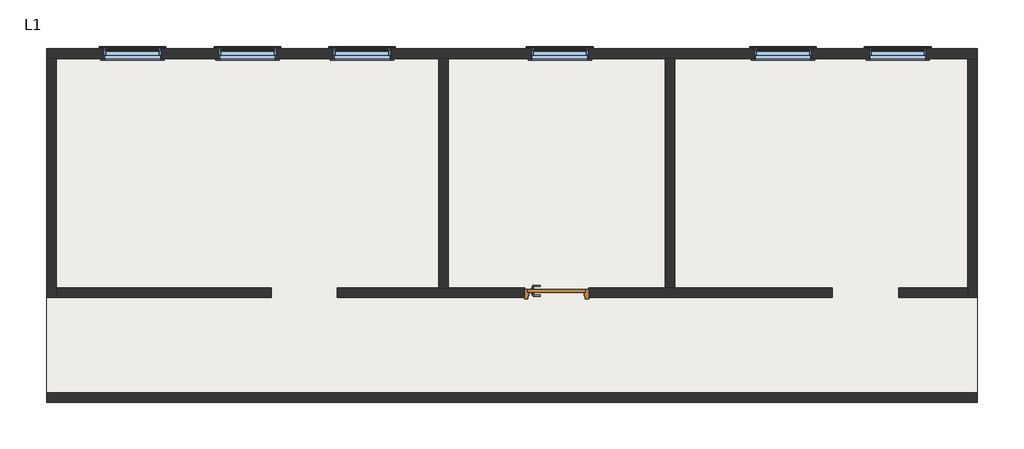
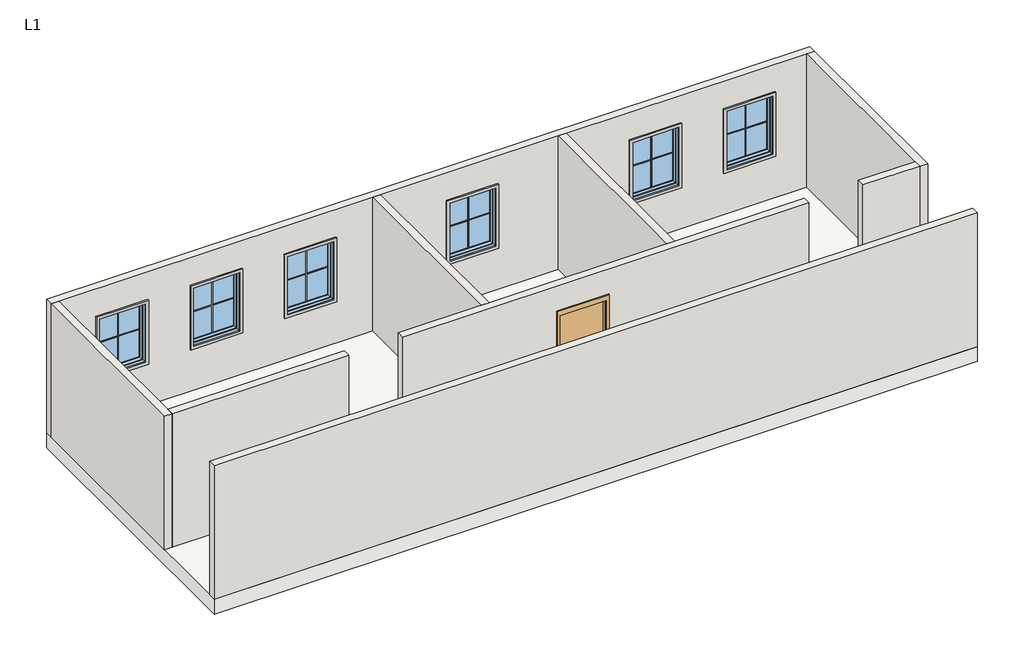
# One storey: 18 proxies, 9 walls, 6 windows, 1 door, 1 slab.
"""IFC4 building model written with IfcOpenShell, lengths in millimetres."""

import ifcopenshell
import ifcopenshell.guid

model = None  # the IFC model being written
_history = None  # IfcOwnerHistory: only IFC2X3 demands one
_inside = {}  # id of a spatial element -> (the spatial element, [elements in it])
_under = {}  # id of a project, library or spatial element -> (it, [spatial elements below it])
_declared = {}  # id of a project -> (the project, [libraries it declares])
_typed = {}  # id of a type object -> (the type object, [elements of that type])
_made_of = {}  # id of a material, layer set ... -> (it, [elements and type objects made of it])


def new_model(schema):
    """Start an empty IFC model of exactly this schema.

    Asked for "IFC4X3", IfcOpenShell would pick the latest addendum, in which some entities
    have other attributes; the version numbers below select the first issue.
    IFC2X3 requires an IfcOwnerHistory on every rooted entity: one is made here for all.
    """
    global model, _history
    if schema == "IFC4X3":
        model = ifcopenshell.file(schema_version=(4, 3, 0, 0))
    else:
        model = ifcopenshell.file(schema=schema)
    _inside.clear()
    _under.clear()
    _declared.clear()
    _typed.clear()
    _made_of.clear()
    _history = None
    if model.schema == "IFC2X3":
        org = make("IfcOrganization", Name="unknown")
        user = make(
            "IfcPersonAndOrganization",
            ThePerson=make("IfcPerson", FamilyName="unknown"),
            TheOrganization=org,
        )
        app = make(
            "IfcApplication",
            ApplicationDeveloper=org,
            Version="unknown",
            ApplicationFullName="unknown",
            ApplicationIdentifier="unknown",
        )
        _history = make(
            "IfcOwnerHistory",
            OwningUser=user,
            OwningApplication=app,
            ChangeAction="ADDED",
            CreationDate=0,
        )
    return model


def make(cls, **values):
    """One entity of the class cls with the attributes given. An attribute that is None is left unset."""
    return model.create_entity(
        cls, **{name: value for name, value in values.items() if value is not None}
    )


def rooted(cls, **values):
    """An entity with a GlobalId (a new one), such as an element, a storey or a relation."""
    return make(cls, GlobalId=ifcopenshell.guid.new(), OwnerHistory=_history, **values)


def si_unit(unit_type, name, prefix=None):
    """IfcSIUnit, for example si_unit("LENGTHUNIT", "METRE", prefix="MILLI")."""
    return make("IfcSIUnit", UnitType=unit_type, Prefix=prefix, Name=name)


def assignment(units):
    """IfcUnitAssignment: the units of a project."""
    return None if units is None else make("IfcUnitAssignment", Units=units)


def point(xyz):
    """IfcCartesianPoint."""
    return None if xyz is None else make("IfcCartesianPoint", Coordinates=xyz)


def direction(xyz):
    """IfcDirection."""
    return None if xyz is None else make("IfcDirection", DirectionRatios=xyz)


def frame(location, z_axis=None, x_axis=None):
    """IfcAxis2Placement3D, a coordinate frame: its origin and axes. An axis left out is left unset."""
    return make(
        "IfcAxis2Placement3D",
        Location=point(location),
        Axis=direction(z_axis),
        RefDirection=direction(x_axis),
    )


def frame_2d(location, x_axis=None):
    """IfcAxis2Placement2D, a coordinate frame in the plane: its origin and x axis."""
    return make(
        "IfcAxis2Placement2D", Location=point(location), RefDirection=direction(x_axis)
    )


def origin():
    """The frame at (0, 0, 0) with its axes left unset."""
    return frame((0.0, 0.0, 0.0))


def origin_with_axes():
    """The frame at (0, 0, 0) with the z axis (0, 0, 1) and the x axis (1, 0, 0) written out."""
    return frame((0.0, 0.0, 0.0), z_axis=(0.0, 0.0, 1.0), x_axis=(1.0, 0.0, 0.0))


def place(relative_to, where):
    """IfcLocalPlacement: puts the frame where relative to a parent placement (None: the world)."""
    return make(
        "IfcLocalPlacement", PlacementRelTo=relative_to, RelativePlacement=where
    )


def context(
    kind, dimensions, precision=None, world=None, true_north=None, identifier=None
):
    """IfcGeometricRepresentationContext, for example the 3D "Model" context."""
    return make(
        "IfcGeometricRepresentationContext",
        ContextIdentifier=identifier,
        ContextType=kind,
        CoordinateSpaceDimension=dimensions,
        Precision=precision,
        WorldCoordinateSystem=world,
        TrueNorth=true_north,
    )


def project(units=None, contexts=None):
    """IfcProject with its units and contexts."""
    return rooted(
        "IfcProject",
        Name="project",
        RepresentationContexts=contexts,
        UnitsInContext=assignment(units),
    )


def spatial(cls, under=None, at=None, **own):
    """A site, building, storey or space (cls), placed at a placement, below another one or the project."""
    s = rooted(cls, ObjectPlacement=at, **own)
    if under is not None:
        _under.setdefault(under.id(), (under, []))[1].append(s)
    return s


def polyline(points):
    """IfcPolyline through the points."""
    return make("IfcPolyline", Points=[point(p) for p in points])


def circle_curve(where, radius):
    """IfcCircle in the frame where."""
    return make("IfcCircle", Position=where, Radius=radius)


def ellipse_curve(where, semi_axis1, semi_axis2):
    """IfcEllipse in the frame where."""
    return make(
        "IfcEllipse", Position=where, SemiAxis1=semi_axis1, SemiAxis2=semi_axis2
    )


def trimmed(basis, trim1, trim2, sense, master):
    """IfcTrimmedCurve: the piece of a basis curve between two trims."""
    return make(
        "IfcTrimmedCurve",
        BasisCurve=basis,
        Trim1=trim1,
        Trim2=trim2,
        SenseAgreement=sense,
        MasterRepresentation=master,
    )


def segment(curve, same_sense, transition):
    """IfcCompositeCurveSegment."""
    return make(
        "IfcCompositeCurveSegment",
        Transition=transition,
        SameSense=same_sense,
        ParentCurve=curve,
    )


def composite_curve(segments, self_intersect=None):
    """IfcCompositeCurve: segments joined end to end."""
    return make("IfcCompositeCurve", Segments=segments, SelfIntersect=self_intersect)


def outline(outer, holes=None, kind="AREA"):
    """IfcArbitraryClosedProfileDef: a profile drawn as a closed curve; with holes, ...WithVoids."""
    if holes is None:
        return make("IfcArbitraryClosedProfileDef", ProfileType=kind, OuterCurve=outer)
    return make(
        "IfcArbitraryProfileDefWithVoids",
        ProfileType=kind,
        OuterCurve=outer,
        InnerCurves=holes,
    )


def extrude(swept, where, along, depth):
    """IfcExtrudedAreaSolid: the profile swept, set in the frame where, extruded along a direction by depth."""
    return make(
        "IfcExtrudedAreaSolid",
        SweptArea=swept,
        Position=where,
        ExtrudedDirection=direction(along),
        Depth=depth,
    )


def faces_of(points, faces, orient=None, outer=None):
    """IfcFace entities. A face is a list of loops; a loop is a list of indices into points, from 0.

    orient and outer hold one flag for each loop. By default every Orientation is true, the
    first loop of a face is its IfcFaceOuterBound and the others are IfcFaceBound.
    """
    made = []
    for i, loops in enumerate(faces):
        bounds = []
        for j, loop in enumerate(loops):
            is_outer = j == 0 if outer is None else outer[i][j]
            bounds.append(
                make(
                    "IfcFaceOuterBound" if is_outer else "IfcFaceBound",
                    Bound=make("IfcPolyLoop", Polygon=[points[k] for k in loop]),
                    Orientation=True if orient is None else orient[i][j],
                )
            )
        made.append(make("IfcFace", Bounds=bounds))
    return made


def faceted_brep(points, faces, orient=None, outer=None, voids=None):
    """IfcFacetedBrep: a solid bounded by flat faces; with voids (closed shells), ...WithVoids."""
    shared = [point(p) for p in points]
    hull = make("IfcClosedShell", CfsFaces=faces_of(shared, faces, orient, outer))
    if voids is None:
        return make("IfcFacetedBrep", Outer=hull)
    return make(
        "IfcFacetedBrepWithVoids",
        Outer=hull,
        Voids=[
            make(cls, CfsFaces=faces_of(shared, fs, o, b)) for cls, fs, o, b in voids
        ],
    )


def shape(context_of_items, identifier, shape_type, items):
    """IfcShapeRepresentation: the items that make up one representation, for example the "Body"."""
    return make(
        "IfcShapeRepresentation",
        ContextOfItems=context_of_items,
        RepresentationIdentifier=identifier,
        RepresentationType=shape_type,
        Items=items,
    )


def source(mapping_origin, context_of_items, identifier, shape_type, items):
    """IfcRepresentationMap: a shape defined once, which mapped items show again and again."""
    return make(
        "IfcRepresentationMap",
        MappingOrigin=mapping_origin,
        MappedRepresentation=shape(context_of_items, identifier, shape_type, items),
    )


def transform(
    local_origin,
    x_axis=None,
    y_axis=None,
    z_axis=None,
    scale=None,
    scale2=None,
    scale3=None,
    uniform=True,
):
    """IfcCartesianTransformationOperator3D, or its non-uniform kind. x_axis, y_axis, z_axis: its Axis1, 2, 3."""
    if uniform:
        return make(
            "IfcCartesianTransformationOperator3D",
            Axis1=direction(x_axis),
            Axis2=direction(y_axis),
            LocalOrigin=point(local_origin),
            Scale=scale,
            Axis3=direction(z_axis),
        )
    return make(
        "IfcCartesianTransformationOperator3DnonUniform",
        Axis1=direction(x_axis),
        Axis2=direction(y_axis),
        LocalOrigin=point(local_origin),
        Scale=scale,
        Axis3=direction(z_axis),
        Scale2=scale2,
        Scale3=scale3,
    )


def mapped(mapping_source, mapping_target):
    """IfcMappedItem: shows the shape of a source again, moved by a transform."""
    return make(
        "IfcMappedItem", MappingSource=mapping_source, MappingTarget=mapping_target
    )


def made_of(thing, what):
    """Note that an element or type object is made of a material, layer set ...; save() writes the relation."""
    if what is not None:
        _made_of.setdefault(what.id(), (what, []))[1].append(thing)
    return thing


def element(
    cls,
    number,
    at=None,
    inside=None,
    cuts=None,
    type_object=None,
    material=None,
    context=None,
    identifier="Body",
    shape_type=None,
    held_by="IfcProductDefinitionShape",
    body=None,
    shapes=None,
    **own,
):
    """One element of the class cls, such as IfcWall. Its Tag is "e" and its number.

    at: its placement. inside: the storey or other place that contains it. cuts: it is an
    opening in that element (IfcRelVoidsElement). A single representation is given by context,
    identifier, shape_type and body (its items); several are given by shapes. held_by: the class
    of the entity that holds the representations. save() writes the other relations.
    """
    e = rooted(cls, Tag="e%d" % number, ObjectPlacement=at, **own)
    if body is not None:
        shapes = [shape(context, identifier, shape_type, body)]
    if shapes is not None:
        e.Representation = make(held_by, Representations=shapes)
    if inside is not None:
        _inside.setdefault(inside.id(), (inside, []))[1].append(e)
    if cuts is not None:
        rooted(
            "IfcRelVoidsElement", RelatingBuildingElement=cuts, RelatedOpeningElement=e
        )
    if type_object is not None:
        _typed.setdefault(type_object.id(), (type_object, []))[1].append(e)
    return made_of(e, material)


def aggregate(whole, parts):
    """IfcRelAggregates: a whole, such as a stair, and the parts it consists of."""
    return rooted("IfcRelAggregates", RelatingObject=whole, RelatedObjects=parts)


def save(model, path):
    """Write the relations noted so far, then the file.

    IfcRelAggregates (storeys below a building ...), IfcRelContainedInSpatialStructure (elements
    in a storey), IfcRelDefinesByType, IfcRelAssociatesMaterial and IfcRelDeclares: one each for
    every whole, place, type object, material and project.
    """
    for whole, parts in _under.values():
        aggregate(whole, parts)
    for where, things in _inside.values():
        rooted(
            "IfcRelContainedInSpatialStructure",
            RelatedElements=things,
            RelatingStructure=where,
        )
    for kind, things in _typed.values():
        rooted("IfcRelDefinesByType", RelatedObjects=things, RelatingType=kind)
    for what, things in _made_of.values():
        rooted("IfcRelAssociatesMaterial", RelatedObjects=things, RelatingMaterial=what)
    for by, libraries in _declared.values():
        rooted("IfcRelDeclares", RelatingContext=by, RelatedDefinitions=libraries)
    model.write(path)


def plane_surface(at):
    """IfcPlane: the flat surface through the origin of the frame at, square to its z axis."""
    return make("IfcPlane", Position=at)


def cylinder_surface(at, radius):
    """IfcCylindricalSurface: all points at the distance radius from the z axis of the frame at."""
    return make("IfcCylindricalSurface", Position=at, Radius=radius)


def revolved_surface(curve, axis_point, axis_direction):
    """IfcSurfaceOfRevolution: the curve turned about the line through axis_point along axis_direction."""
    return make(
        "IfcSurfaceOfRevolution",
        SweptCurve=make("IfcArbitraryOpenProfileDef", ProfileType="CURVE", Curve=curve),
        AxisPosition=make("IfcAxis1Placement", Location=point(axis_point), Axis=direction(axis_direction)),
    )


def advanced_brep(points, edges, surfaces, faces):
    """IfcAdvancedBrep: a solid bounded by faces that lie on surfaces and meet in shared edges.

    An edge is (start, end): straight between two places in points (the first is 0);
    or (start, end, curve); or (start, end, curve, False) where it runs against its curve.
    A face is (place in surfaces, loops), or (place, loops, False) where it looks against
    its surface's normal. A loop lists edges by number (the first is 1), with a minus sign
    where the edge is run from its end to its start. The first loop is the outer one.
    """
    corners = [point(p) for p in points]
    vertices = [make("IfcVertexPoint", VertexGeometry=c) for c in corners]
    made = []
    for start, end, *more in edges:
        made.append(
            make(
                "IfcEdgeCurve",
                EdgeStart=vertices[start],
                EdgeEnd=vertices[end],
                EdgeGeometry=more[0] if more else make("IfcPolyline", Points=[corners[start], corners[end]]),
                SameSense=more[1] if len(more) > 1 else True,
            )
        )
    hull = []
    for where, loops, *sense in faces:
        bounds = []
        for j, loop in enumerate(loops):
            ring = [make("IfcOrientedEdge", EdgeElement=made[abs(k) - 1], Orientation=k > 0) for k in loop]
            bounds.append(
                make(
                    "IfcFaceOuterBound" if j == 0 else "IfcFaceBound",
                    Bound=make("IfcEdgeLoop", EdgeList=ring),
                    Orientation=True,
                )
            )
        hull.append(make("IfcAdvancedFace", Bounds=bounds, FaceSurface=surfaces[where], SameSense=sense[0] if sense else True))
    return make("IfcAdvancedBrep", Outer=make("IfcClosedShell", CfsFaces=hull))


def m_muntin_pattern_2x2_m_muntin_pattern_2x2_ad852c99(model_context):
    return source(origin(), model_context, "Body", "SweptSolid", [
        extrude(outline(polyline([(568.25, -6.35), (568.25, -411.9), (555.55, -411.9), (555.55, -6.35), (0.0, -6.35), (0.0, 6.35), (555.55, 6.35), (555.55, 411.9), (568.25, 411.9), (568.25, 6.35), (1123.8, 6.35), (1123.8, -6.35), (568.25, -6.35)])), frame((0.0, -22.225, 0.0), z_axis=(0.0, 1.0, 0.0), x_axis=(0.0, 0.0, 1.0)), (0.0, 0.0, 1.0), 12.7),
        extrude(outline(polyline([(568.25, -6.35), (568.25, -411.9), (555.55, -411.9), (555.55, -6.35), (0.0, -6.35), (0.0, 6.35), (555.55, 6.35), (555.55, 411.9), (568.25, 411.9), (568.25, 6.35), (1123.8, 6.35), (1123.8, -6.35), (568.25, -6.35)])), frame((0.0, 9.525, 0.0), z_axis=(0.0, 1.0, 0.0), x_axis=(0.0, 0.0, 1.0)), (0.0, 0.0, 1.0), 12.7),
    ])


def m_trim_window_exterior_flat_with_sill_71544b40(model_context):
    return source(origin(), model_context, "Body", "SweptSolid", [
        extrude(outline(polyline([(510.0, -1220.4323709), (510.0, -1280.4323709), (-510.0, -1280.4323709), (-510.0, -1220.4323709), (510.0, -1220.4323709)])), origin_with_axes(), (0.0, 0.0, 1.0), 19.05),
        extrude(outline(polyline([(-1230.0, 38.1), (-1202.4580645, 38.1), (-1200.0, 19.05), (-1200.0, 0.0), (-1220.4323709, 0.0), (-1220.4323709, 19.05), (-1230.0, 19.05), (-1230.0, 38.1)])), frame((-522.7, 0.0, 0.0), z_axis=(1.0, 0.0, 0.0), x_axis=(0.0, 1.0, 0.0)), (0.0, 0.0, 1.0), 1045.4),
        extrude(outline(polyline([(-510.0, 60.0), (510.0, 60.0), (510.0, -1200.0), (450.0, -1200.0), (450.0, 0.0), (-450.0, 0.0), (-450.0, -1200.0), (-510.0, -1200.0), (-510.0, 60.0)])), origin_with_axes(), (0.0, 0.0, 1.0), 19.05),
    ])


def m_trim_window_interior_flat_picture_frame_24fe8ef8(model_context):
    return source(origin(), model_context, "Body", "SweptSolid", [
        extrude(outline(polyline([(497.3, 47.3), (497.3, -1247.3), (-497.3, -1247.3), (-497.3, 47.3), (497.3, 47.3)]), holes=[polyline([(437.3, -12.7), (-437.3, -12.7), (-437.3, -1187.3), (437.3, -1187.3), (437.3, -12.7)])]), origin_with_axes(), (0.0, 0.0, 1.0), 30.0),
    ])


def m_door_passage_single_flush_900_x_2100mm_f70d95c9(model_context):
    return source(origin(), model_context, "Body", "SolidModel", [
        advanced_brep(
        [(-384.990625, 3.35, 1000.0), (-364.990625, 3.35, 1000.0), (-364.990625, -26.65, 1000.0), (-384.990625, -26.65, 1000.0), (-359.990625, -31.65, 1000.0), (-359.990625, -51.65, 1000.0), (-254.990625, -51.65, 1000.0), (-254.990625, -31.65, 1000.0)],
        [
            (0, 1, circle_curve(frame((-374.990625, 3.35, 1000.0), z_axis=(0.0, 1.0, 0.0), x_axis=(1.0, 0.0, 0.0)), 10.0)),
            (1, 0, circle_curve(frame((-374.990625, 3.35, 1000.0), z_axis=(0.0, 1.0, 0.0), x_axis=(1.0, 0.0, 0.0)), 10.0)),
            (1, 2),
            (2, 3, circle_curve(frame((-374.990625, -26.65, 1000.0), z_axis=(0.0, 1.0, 0.0), x_axis=(1.0, 0.0, 0.0)), 10.0)),
            (3, 0),
            (3, 2, circle_curve(frame((-374.990625, -26.65, 1000.0), z_axis=(0.0, 1.0, 0.0), x_axis=(1.0, 0.0, 0.0)), 10.0)),
            (4, 5, circle_curve(frame((-359.990625, -41.65, 1000.0), z_axis=(-1.0, 0.0, 0.0), x_axis=(0.0, 1.0, 0.0)), 10.0)),
            (5, 3, circle_curve(frame((-359.990625, -26.65, 1000.0), z_axis=(0.0, 0.0, -1.0), x_axis=(-1.0, 0.0, 0.0)), 25.0)),
            (2, 4, circle_curve(frame((-359.990625, -26.65, 1000.0), z_axis=(0.0, 0.0, 1.0), x_axis=(-1.0, 0.0, 0.0)), 5.0)),
            (5, 4, circle_curve(frame((-359.990625, -41.65, 1000.0), z_axis=(-1.0, 0.0, 0.0), x_axis=(0.0, 1.0, 0.0)), 10.0)),
            (6, 7, circle_curve(frame((-254.990625, -41.65, 1000.0), z_axis=(1.0, 0.0, 0.0), x_axis=(0.0, 1.0, 0.0)), 10.0)),
            (7, 6, circle_curve(frame((-254.990625, -41.65, 1000.0), z_axis=(1.0, 0.0, 0.0), x_axis=(0.0, 1.0, 0.0)), 10.0)),
            (4, 7),
            (6, 5),
        ],
        [
            plane_surface(frame((-374.990625, 3.35, 1000.0), z_axis=(0.0, 1.0, 0.0), x_axis=(0.0, 0.0, 1.0))),
            cylinder_surface(frame((-374.990625, 3.35, 1000.0), z_axis=(0.0, 1.0, 0.0), x_axis=(1.0, 0.0, 0.0)), 10.0),
            revolved_surface(trimmed(ellipse_curve(frame((-374.990625, -26.65, 1000.0), z_axis=(0.0, -1.0, 0.0), x_axis=(1.0, 0.0, 0.0)), 10.0, 10.0), [point((-384.990625, -26.65, 1000.0))], [point((-364.990625, -26.65, 1000.0))], True, "CARTESIAN"), (-359.990625, -26.65, 1000.0), (0.0, 0.0, -1.0)),
            revolved_surface(trimmed(ellipse_curve(frame((-374.990625, -26.65, 1000.0), z_axis=(0.0, -1.0, 0.0), x_axis=(1.0, 0.0, 0.0)), 10.0, 10.0), [point((-364.990625, -26.65, 1000.0))], [point((-384.990625, -26.65, 1000.0))], True, "CARTESIAN"), (-359.990625, -26.65, 1000.0), (0.0, 0.0, -1.0)),
            plane_surface(frame((-254.990625, -41.65, 1000.0), z_axis=(1.0, 0.0, 0.0), x_axis=(0.0, 0.0, 1.0))),
            cylinder_surface(frame((-359.990625, -41.65, 1000.0), z_axis=(-1.0, 0.0, 0.0), x_axis=(0.0, 1.0, 0.0)), 10.0),
        ],
        [
            (0, [[1, 2]]),
            (1, [[3, 4, 5, -2]]),
            (1, [[-5, 6, -3, -1]]),
            (2, [[7, 8, -4, 9]]),
            (3, [[10, -9, -6, -8]]),
            (4, [[11, 12]]),
            (5, [[13, -11, 14, -7]]),
            (5, [[-14, -12, -13, -10]]),
        ],
    ),
        extrude(outline(composite_curve([segment(trimmed(circle_curve(frame_2d((1000.0, -377.490625)), 30.0), [point((1000.0, -407.490625))], [point((1000.0, -347.490625))], False, "CARTESIAN"), True, "CONTINUOUS"), segment(trimmed(circle_curve(frame_2d((1000.0, -377.490625)), 30.0), [point((1000.0, -347.490625))], [point((1000.0, -407.490625))], False, "CARTESIAN"), True, "CONTINUOUS")], self_intersect=False)), frame((0.0, 3.35, 0.0), z_axis=(0.0, 1.0, 0.0), x_axis=(0.0, 0.0, 1.0)), (0.0, 0.0, 1.0), 8.0),
        advanced_brep(
        [(-384.990625, 64.35, 1000.0), (-364.990625, 64.35, 1000.0), (-384.990625, 94.35, 1000.0), (-364.990625, 94.35, 1000.0), (-359.990625, 99.35, 1000.0), (-359.990625, 119.35, 1000.0), (-254.990625, 119.35, 1000.0), (-254.990625, 99.35, 1000.0)],
        [
            (0, 1, circle_curve(frame((-374.990625, 64.35, 1000.0), z_axis=(0.0, -1.0, 0.0), x_axis=(1.0, 0.0, 0.0)), 10.0)),
            (1, 0, circle_curve(frame((-374.990625, 64.35, 1000.0), z_axis=(0.0, -1.0, 0.0), x_axis=(1.0, 0.0, 0.0)), 10.0)),
            (0, 2),
            (2, 3, circle_curve(frame((-374.990625, 94.35, 1000.0), z_axis=(0.0, -1.0, 0.0), x_axis=(1.0, 0.0, 0.0)), 10.0)),
            (3, 1),
            (3, 2, circle_curve(frame((-374.990625, 94.35, 1000.0), z_axis=(0.0, -1.0, 0.0), x_axis=(1.0, 0.0, 0.0)), 10.0)),
            (4, 3, circle_curve(frame((-359.990625, 94.35, 1000.0), z_axis=(0.0, 0.0, 1.0), x_axis=(-1.0, 0.0, 0.0)), 5.0)),
            (2, 5, circle_curve(frame((-359.990625, 94.35, 1000.0), z_axis=(0.0, 0.0, -1.0), x_axis=(-1.0, 0.0, 0.0)), 25.0)),
            (5, 4, circle_curve(frame((-359.990625, 109.35, 1000.0), z_axis=(-1.0, 0.0, 0.0), x_axis=(0.0, -1.0, 0.0)), 10.0)),
            (4, 5, circle_curve(frame((-359.990625, 109.35, 1000.0), z_axis=(-1.0, 0.0, 0.0), x_axis=(0.0, -1.0, 0.0)), 10.0)),
            (6, 7, circle_curve(frame((-254.990625, 109.35, 1000.0), z_axis=(1.0, 0.0, 0.0), x_axis=(0.0, -1.0, 0.0)), 10.0)),
            (7, 6, circle_curve(frame((-254.990625, 109.35, 1000.0), z_axis=(1.0, 0.0, 0.0), x_axis=(0.0, -1.0, 0.0)), 10.0)),
            (5, 6),
            (7, 4),
        ],
        [
            plane_surface(frame((-374.990625, 64.35, 1000.0), z_axis=(0.0, -1.0, 0.0), x_axis=(0.0, 0.0, 1.0))),
            cylinder_surface(frame((-374.990625, 64.35, 1000.0), z_axis=(0.0, -1.0, 0.0), x_axis=(1.0, 0.0, 0.0)), 10.0),
            revolved_surface(trimmed(ellipse_curve(frame((-374.990625, 94.35, 1000.0), z_axis=(0.0, -1.0, 0.0), x_axis=(1.0, 0.0, 0.0)), 10.0, 10.0), [point((-384.990625, 94.35, 1000.0))], [point((-364.990625, 94.35, 1000.0))], True, "CARTESIAN"), (-359.990625, 94.35, 1000.0), (0.0, 0.0, -1.0)),
            revolved_surface(trimmed(ellipse_curve(frame((-374.990625, 94.35, 1000.0), z_axis=(0.0, -1.0, 0.0), x_axis=(1.0, 0.0, 0.0)), 10.0, 10.0), [point((-364.990625, 94.35, 1000.0))], [point((-384.990625, 94.35, 1000.0))], True, "CARTESIAN"), (-359.990625, 94.35, 1000.0), (0.0, 0.0, -1.0)),
            plane_surface(frame((-254.990625, 109.35, 1000.0), z_axis=(1.0, 0.0, 0.0), x_axis=(0.0, 0.0, 1.0))),
            cylinder_surface(frame((-359.990625, 109.35, 1000.0), z_axis=(-1.0, 0.0, 0.0), x_axis=(0.0, -1.0, 0.0)), 10.0),
        ],
        [
            (0, [[1, 2]]),
            (1, [[-1, 3, 4, 5]]),
            (1, [[-2, -5, 6, -3]]),
            (2, [[7, -4, 8, 9]]),
            (3, [[-8, -6, -7, 10]]),
            (4, [[11, 12]]),
            (5, [[-9, 13, -12, 14]]),
            (5, [[-10, -14, -11, -13]]),
        ],
    ),
        extrude(outline(composite_curve([segment(trimmed(circle_curve(frame_2d((1000.0, -377.490625)), 30.0), [point((1000.0, -407.490625))], [point((1000.0, -347.490625))], False, "CARTESIAN"), True, "CONTINUOUS"), segment(trimmed(circle_curve(frame_2d((1000.0, -377.490625)), 30.0), [point((1000.0, -347.490625))], [point((1000.0, -407.490625))], False, "CARTESIAN"), True, "CONTINUOUS")], self_intersect=False)), frame((0.0, 56.35, 0.0), z_axis=(0.0, 1.0, 0.0), x_axis=(0.0, 0.0, 1.0)), (0.0, 0.0, 1.0), 8.0),
        extrude(outline(polyline([(450.0, 11.35), (-450.0, 11.35), (-450.0, 56.35), (450.0, 56.35), (450.0, 11.35)])), origin_with_axes(), (0.0, 0.0, 1.0), 2100.0),
        faceted_brep([(450.0, 6.5875, 0.0), (450.0, 56.35, 0.0), (500.0, 56.35, 0.0), (500.0, -93.65, 0.0), (450.0, -93.65, 0.0), (450.0, -44.4375, 0.0), (434.125, -44.4375, 0.0), (434.125, 6.5875, 0.0), (450.0, 6.5875, 2100.0), (450.0, 56.35, 2100.0), (-450.0, 56.35, 2100.0), (-450.0, 56.35, 0.0), (-500.0, 56.35, 0.0), (-500.0, 56.35, 2200.0), (500.0, 56.35, 2200.0), (500.0, -93.65, 2200.0), (-500.0, -93.65, 2200.0), (-500.0, -93.65, 0.0), (-450.0, -93.65, 0.0), (-450.0, -93.65, 2100.0), (450.0, -93.65, 2100.0), (450.0, -44.4375, 2100.0), (-450.0, -44.4375, 2100.0), (-450.0, -44.4375, 0.0), (-434.125, -44.4375, 0.0), (-434.125, -44.4375, 2084.125), (434.125, -44.4375, 2084.125), (434.125, 6.5875, 2084.125), (-434.125, 6.5875, 2084.125), (-434.125, 6.5875, 0.0), (-450.0, 6.5875, 0.0), (-450.0, 6.5875, 2100.0)], [[[0, 1, 2, 3, 4, 5, 6, 7]], [[1, 0, 8, 9]], [[2, 1, 9, 10, 11, 12, 13, 14]], [[3, 2, 14, 15]], [[4, 3, 15, 16, 17, 18, 19, 20]], [[5, 4, 20, 21]], [[6, 5, 21, 22, 23, 24, 25, 26]], [[7, 6, 26, 27]], [[0, 7, 27, 28, 29, 30, 31, 8]], [[9, 8, 31, 10]], [[20, 19, 22, 21]], [[26, 25, 28, 27]], [[12, 11, 30, 29, 24, 23, 18, 17]], [[11, 10, 31, 30]], [[13, 12, 17, 16]], [[19, 18, 23, 22]], [[25, 24, 29, 28]], [[15, 14, 13, 16]]]),
    ])


def m_window_fixed_900_x_1200mm_f2c8dc95(model_context):
    return source(origin(), model_context, "Body", "SolidModel", [
        faceted_brep([(450.0, -20.25, 2100.0), (450.0, 94.05, 2100.0), (-450.0, 94.05, 2100.0), (-450.0, -20.25, 2100.0), (-450.0, 94.05, 900.0), (-450.0, -20.25, 900.0), (450.0, 94.05, 900.0), (450.0, -20.25, 900.0), (418.25, -20.25, 2068.25), (418.25, -20.25, 931.75), (-418.25, -20.25, 931.75), (-418.25, -20.25, 2068.25), (-437.3, 94.05, 2087.3), (-437.3, 94.05, 912.7), (437.3, 94.05, 912.7), (437.3, 94.05, 2087.3), (418.25, 43.25, 2068.25), (-418.25, 43.25, 2068.25), (437.3, 43.25, 2087.3), (-437.3, 43.25, 2087.3), (-418.25, 43.25, 931.75), (-437.3, 43.25, 912.7), (418.25, 43.25, 931.75), (437.3, 43.25, 912.7)], [[[0, 1, 2, 3]], [[3, 2, 4, 5]], [[5, 4, 6, 7]], [[3, 5, 7, 0], [8, 9, 10, 11]], [[7, 6, 1, 0]], [[1, 6, 4, 2], [12, 13, 14, 15]], [[16, 8, 11, 17]], [[15, 18, 19, 12]], [[17, 11, 10, 20]], [[12, 19, 21, 13]], [[20, 10, 9, 22]], [[13, 21, 23, 14]], [[22, 9, 8, 16]], [[18, 23, 21, 19], [17, 20, 22, 16]], [[14, 23, 18, 15]]]),
        extrude(outline(polyline([(2100.0, -450.0), (900.0, -450.0), (900.0, 450.0), (2100.0, 450.0), (2100.0, -450.0)]), holes=[polyline([(2087.3, 437.3), (912.7, 437.3), (912.7, -437.3), (2087.3, -437.3), (2087.3, 437.3)])]), frame((0.0, -75.0, 0.0), z_axis=(0.0, 1.0, 0.0), x_axis=(0.0, 0.0, 1.0)), (0.0, 0.0, 1.0), 54.75),
        extrude(outline(polyline([(912.7, 437.3), (2087.3, 437.3), (2087.3, -437.3), (912.7, -437.3), (912.7, 437.3)]), holes=[polyline([(938.1, -411.9), (2061.9, -411.9), (2061.9, 411.9), (938.1, 411.9), (938.1, -411.9)])]), frame((0.0, 43.25, 0.0), z_axis=(0.0, 1.0, 0.0), x_axis=(0.0, 0.0, 1.0)), (0.0, 0.0, 1.0), 44.45),
        extrude(outline(polyline([(411.9, 75.0), (411.9, 68.65), (-411.9, 68.65), (-411.9, 75.0), (411.9, 75.0)])), frame((0.0, 0.0, 938.1), z_axis=(0.0, 0.0, 1.0), x_axis=(1.0, 0.0, 0.0)), (0.0, 0.0, 1.0), 1123.8),
        extrude(outline(polyline([(-411.9, 55.95), (-411.9, 62.3), (411.9, 62.3), (411.9, 55.95), (-411.9, 55.95)])), frame((0.0, 0.0, 938.1), z_axis=(0.0, 0.0, 1.0), x_axis=(1.0, 0.0, 0.0)), (0.0, 0.0, 1.0), 1123.8),
    ])


model = new_model("IFC4")

# Units and contexts
model_context = context("Model", 3, world=origin())
ifc_project = project(units=[si_unit("LENGTHUNIT", "METRE", prefix="MILLI")], contexts=[model_context])

# Site, building, storey
site = spatial("IfcSite", under=ifc_project)
building = spatial("IfcBuilding", under=site)
storey = spatial("IfcBuildingStorey", under=building, Name="L1", Elevation=0.0)

# Proxies
placement = place(None, origin())
m_muntin_pattern_2x2_m_muntin_pattern_2x2_shape = m_muntin_pattern_2x2_m_muntin_pattern_2x2_ad852c99(model_context)
element("IfcBuildingElementProxy", 1, Name="M_Muntin Pattern_2x2 : M_Muntin Pattern_2x2", ObjectType="M_Muntin Pattern_2x2 : M_Muntin Pattern_2x2", at=placement, inside=storey, context=model_context, shape_type="MappedRepresentation", body=[
    mapped(m_muntin_pattern_2x2_m_muntin_pattern_2x2_shape, transform((1675.0, 3815.475, 938.1), x_axis=(-1.0, 0.0, 0.0), y_axis=(0.0, -1.0, 0.0), z_axis=(0.0, 0.0, 1.0))),
])
element("IfcBuildingElementProxy", 2, Name="M_Muntin Pattern_2x2 : M_Muntin Pattern_2x2", ObjectType="M_Muntin Pattern_2x2 : M_Muntin Pattern_2x2", at=placement, inside=storey, context=model_context, shape_type="MappedRepresentation", body=[
    mapped(m_muntin_pattern_2x2_m_muntin_pattern_2x2_shape, transform((-1425.0, 3815.475, 938.1), x_axis=(-1.0, 0.0, 0.0), y_axis=(0.0, -1.0, 0.0), z_axis=(0.0, 0.0, 1.0))),
])
element("IfcBuildingElementProxy", 3, Name="M_Muntin Pattern_2x2 : M_Muntin Pattern_2x2", ObjectType="M_Muntin Pattern_2x2 : M_Muntin Pattern_2x2", at=placement, inside=storey, context=model_context, shape_type="MappedRepresentation", body=[
    mapped(m_muntin_pattern_2x2_m_muntin_pattern_2x2_shape, transform((-3225.0, 3815.475, 938.1), x_axis=(-1.0, 0.0, 0.0), y_axis=(0.0, -1.0, 0.0), z_axis=(0.0, 0.0, 1.0))),
])
element("IfcBuildingElementProxy", 4, Name="M_Muntin Pattern_2x2 : M_Muntin Pattern_2x2", ObjectType="M_Muntin Pattern_2x2 : M_Muntin Pattern_2x2", at=placement, inside=storey, context=model_context, shape_type="MappedRepresentation", body=[
    mapped(m_muntin_pattern_2x2_m_muntin_pattern_2x2_shape, transform((-5025.0, 3815.475, 938.1), x_axis=(-1.0, 0.0, 0.0), y_axis=(0.0, -1.0, 0.0), z_axis=(0.0, 0.0, 1.0))),
])
element("IfcBuildingElementProxy", 5, Name="M_Muntin Pattern_2x2 : M_Muntin Pattern_2x2", ObjectType="M_Muntin Pattern_2x2 : M_Muntin Pattern_2x2", at=placement, inside=storey, context=model_context, shape_type="MappedRepresentation", body=[
    mapped(m_muntin_pattern_2x2_m_muntin_pattern_2x2_shape, transform((5175.0, 3815.475, 938.1), x_axis=(-1.0, 0.0, 0.0), y_axis=(0.0, -1.0, 0.0), z_axis=(0.0, 0.0, 1.0))),
])
element("IfcBuildingElementProxy", 6, Name="M_Muntin Pattern_2x2 : M_Muntin Pattern_2x2", ObjectType="M_Muntin Pattern_2x2 : M_Muntin Pattern_2x2", at=placement, inside=storey, context=model_context, shape_type="MappedRepresentation", body=[
    mapped(m_muntin_pattern_2x2_m_muntin_pattern_2x2_shape, transform((6975.0, 3815.475, 938.1), x_axis=(-1.0, 0.0, 0.0), y_axis=(0.0, -1.0, 0.0), z_axis=(0.0, 0.0, 1.0))),
])
m_trim_window_exterior_flat_with_sill_shape = m_trim_window_exterior_flat_with_sill_71544b40(model_context)
element("IfcBuildingElementProxy", 7, Name="M_Trim-Window-Exterior-Flat : with Sill", ObjectType="M_Trim-Window-Exterior-Flat : with Sill", at=placement, inside=storey, context=model_context, shape_type="MappedRepresentation", body=[
    mapped(m_trim_window_exterior_flat_with_sill_shape, transform((1675.0, 3825.0, 2100.0), x_axis=(-1.0, 0.0, 0.0), y_axis=(0.0, 0.0, 1.0), z_axis=(0.0, 1.0, 0.0))),
])
element("IfcBuildingElementProxy", 8, Name="M_Trim-Window-Exterior-Flat : with Sill", ObjectType="M_Trim-Window-Exterior-Flat : with Sill", at=placement, inside=storey, context=model_context, shape_type="MappedRepresentation", body=[
    mapped(m_trim_window_exterior_flat_with_sill_shape, transform((-1425.0, 3825.0, 2100.0), x_axis=(-1.0, 0.0, 0.0), y_axis=(0.0, 0.0, 1.0), z_axis=(0.0, 1.0, 0.0))),
])
element("IfcBuildingElementProxy", 9, Name="M_Trim-Window-Exterior-Flat : with Sill", ObjectType="M_Trim-Window-Exterior-Flat : with Sill", at=placement, inside=storey, context=model_context, shape_type="MappedRepresentation", body=[
    mapped(m_trim_window_exterior_flat_with_sill_shape, transform((-3225.0, 3825.0, 2100.0), x_axis=(-1.0, 0.0, 0.0), y_axis=(0.0, 0.0, 1.0), z_axis=(0.0, 1.0, 0.0))),
])
element("IfcBuildingElementProxy", 10, Name="M_Trim-Window-Exterior-Flat : with Sill", ObjectType="M_Trim-Window-Exterior-Flat : with Sill", at=placement, inside=storey, context=model_context, shape_type="MappedRepresentation", body=[
    mapped(m_trim_window_exterior_flat_with_sill_shape, transform((-5025.0, 3825.0, 2100.0), x_axis=(-1.0, 0.0, 0.0), y_axis=(0.0, 0.0, 1.0), z_axis=(0.0, 1.0, 0.0))),
])
element("IfcBuildingElementProxy", 11, Name="M_Trim-Window-Exterior-Flat : with Sill", ObjectType="M_Trim-Window-Exterior-Flat : with Sill", at=placement, inside=storey, context=model_context, shape_type="MappedRepresentation", body=[
    mapped(m_trim_window_exterior_flat_with_sill_shape, transform((5175.0, 3825.0, 2100.0), x_axis=(-1.0, 0.0, 0.0), y_axis=(0.0, 0.0, 1.0), z_axis=(0.0, 1.0, 0.0))),
])
element("IfcBuildingElementProxy", 12, Name="M_Trim-Window-Exterior-Flat : with Sill", ObjectType="M_Trim-Window-Exterior-Flat : with Sill", at=placement, inside=storey, context=model_context, shape_type="MappedRepresentation", body=[
    mapped(m_trim_window_exterior_flat_with_sill_shape, transform((6975.0, 3825.0, 2100.0), x_axis=(-1.0, 0.0, 0.0), y_axis=(0.0, 0.0, 1.0), z_axis=(0.0, 1.0, 0.0))),
])
m_trim_window_interior_flat_picture_frame_shape = m_trim_window_interior_flat_picture_frame_24fe8ef8(model_context)
element("IfcBuildingElementProxy", 13, Name="M_Trim-Window-Interior-Flat : Picture Frame", ObjectType="M_Trim-Window-Interior-Flat : Picture Frame", at=placement, inside=storey, context=model_context, shape_type="MappedRepresentation", body=[
    mapped(m_trim_window_interior_flat_picture_frame_shape, transform((1675.0, 3675.0, 2100.0), x_axis=(1.0, 0.0, 0.0), y_axis=(0.0, 0.0, 1.0), z_axis=(0.0, -1.0, 0.0))),
])
element("IfcBuildingElementProxy", 14, Name="M_Trim-Window-Interior-Flat : Picture Frame", ObjectType="M_Trim-Window-Interior-Flat : Picture Frame", at=placement, inside=storey, context=model_context, shape_type="MappedRepresentation", body=[
    mapped(m_trim_window_interior_flat_picture_frame_shape, transform((-1425.0, 3675.0, 2100.0), x_axis=(1.0, 0.0, 0.0), y_axis=(0.0, 0.0, 1.0), z_axis=(0.0, -1.0, 0.0))),
])
element("IfcBuildingElementProxy", 15, Name="M_Trim-Window-Interior-Flat : Picture Frame", ObjectType="M_Trim-Window-Interior-Flat : Picture Frame", at=placement, inside=storey, context=model_context, shape_type="MappedRepresentation", body=[
    mapped(m_trim_window_interior_flat_picture_frame_shape, transform((-3225.0, 3675.0, 2100.0), x_axis=(1.0, 0.0, 0.0), y_axis=(0.0, 0.0, 1.0), z_axis=(0.0, -1.0, 0.0))),
])
element("IfcBuildingElementProxy", 16, Name="M_Trim-Window-Interior-Flat : Picture Frame", ObjectType="M_Trim-Window-Interior-Flat : Picture Frame", at=placement, inside=storey, context=model_context, shape_type="MappedRepresentation", body=[
    mapped(m_trim_window_interior_flat_picture_frame_shape, transform((-5025.0, 3675.0, 2100.0), x_axis=(1.0, 0.0, 0.0), y_axis=(0.0, 0.0, 1.0), z_axis=(0.0, -1.0, 0.0))),
])
element("IfcBuildingElementProxy", 17, Name="M_Trim-Window-Interior-Flat : Picture Frame", ObjectType="M_Trim-Window-Interior-Flat : Picture Frame", at=placement, inside=storey, context=model_context, shape_type="MappedRepresentation", body=[
    mapped(m_trim_window_interior_flat_picture_frame_shape, transform((5175.0, 3675.0, 2100.0), x_axis=(1.0, 0.0, 0.0), y_axis=(0.0, 0.0, 1.0), z_axis=(0.0, -1.0, 0.0))),
])
element("IfcBuildingElementProxy", 18, Name="M_Trim-Window-Interior-Flat : Picture Frame", ObjectType="M_Trim-Window-Interior-Flat : Picture Frame", at=placement, inside=storey, context=model_context, shape_type="MappedRepresentation", body=[
    mapped(m_trim_window_interior_flat_picture_frame_shape, transform((6975.0, 3675.0, 2100.0), x_axis=(1.0, 0.0, 0.0), y_axis=(0.0, 0.0, 1.0), z_axis=(0.0, -1.0, 0.0))),
])

# Door
m_door_passage_single_flush_900_x_2100mm_shape = m_door_passage_single_flush_900_x_2100mm_f70d95c9(model_context)
element("IfcDoor", 19, ObjectType="M_Door-Passage-Single-Flush : 900 x 2100mm", at=placement, inside=storey, context=model_context, shape_type="MappedRepresentation", body=[
    mapped(m_door_passage_single_flush_900_x_2100mm_shape, transform((1625.0, -6.35, 0.0), x_axis=(1.0, 0.0, 0.0), y_axis=(0.0, 1.0, 0.0), z_axis=(0.0, 0.0, 1.0))),
])

# Slab
element("IfcSlab", 20, ObjectType="Generic 300mm", at=placement, inside=storey, context=model_context, shape_type="SweptSolid", body=[
    extrude(outline(polyline([(8225.0, 3825.0), (8225.0, -1725.0), (-6375.0, -1725.0), (-6375.0, 3825.0), (8225.0, 3825.0)])), frame((0.0, 0.0, -300.0), z_axis=(0.0, 0.0, 1.0), x_axis=(1.0, 0.0, 0.0)), (0.0, 0.0, 1.0), 300.0),
])

# Walls
element("IfcWall", 21, ObjectType="Generic - 150mm", at=placement, inside=storey, context=model_context, shape_type="SweptSolid", body=[
    extrude(outline(polyline([(-75.0, 3675.0), (-75.0, 75.0), (-225.0, 75.0), (-225.0, 3675.0), (-75.0, 3675.0)])), origin_with_axes(), (0.0, 0.0, 1.0), 2700.0),
])
element("IfcWall", 22, ObjectType="Generic - 150mm", at=placement, inside=storey, context=model_context, shape_type="Brep", body=[
    faceted_brep([(-6375.0, 3675.0, 0.0), (-6225.0, 3675.0, 0.0), (-225.0, 3675.0, 0.0), (-75.0, 3675.0, 0.0), (3325.0, 3675.0, 0.0), (3475.0, 3675.0, 0.0), (8075.0, 3675.0, 0.0), (8225.0, 3675.0, 0.0), (8225.0, 3675.0, 2700.0), (8075.0, 3675.0, 2700.0), (3475.0, 3675.0, 2700.0), (3325.0, 3675.0, 2700.0), (-75.0, 3675.0, 2700.0), (-225.0, 3675.0, 2700.0), (-6225.0, 3675.0, 2700.0), (-6375.0, 3675.0, 2700.0), (2125.0, 3675.0, 2100.0), (2125.0, 3675.0, 900.0), (1225.0, 3675.0, 900.0), (1225.0, 3675.0, 2100.0), (-975.0, 3675.0, 2100.0), (-975.0, 3675.0, 900.0), (-1875.0, 3675.0, 900.0), (-1875.0, 3675.0, 2100.0), (-2775.0, 3675.0, 2100.0), (-2775.0, 3675.0, 900.0), (-3675.0, 3675.0, 900.0), (-3675.0, 3675.0, 2100.0), (-4575.0, 3675.0, 2100.0), (-4575.0, 3675.0, 900.0), (-5475.0, 3675.0, 900.0), (-5475.0, 3675.0, 2100.0), (5625.0, 3675.0, 2100.0), (5625.0, 3675.0, 900.0), (4725.0, 3675.0, 900.0), (4725.0, 3675.0, 2100.0), (7425.0, 3675.0, 2100.0), (7425.0, 3675.0, 900.0), (6525.0, 3675.0, 900.0), (6525.0, 3675.0, 2100.0), (-6375.0, 3825.0, 0.0), (-6375.0, 3825.0, 2700.0), (8225.0, 3825.0, 2700.0), (8225.0, 3825.0, 0.0), (2125.0, 3825.0, 2100.0), (1225.0, 3825.0, 2100.0), (1225.0, 3825.0, 900.0), (2125.0, 3825.0, 900.0), (-975.0, 3825.0, 2100.0), (-1875.0, 3825.0, 2100.0), (-1875.0, 3825.0, 900.0), (-975.0, 3825.0, 900.0), (-2775.0, 3825.0, 2100.0), (-3675.0, 3825.0, 2100.0), (-3675.0, 3825.0, 900.0), (-2775.0, 3825.0, 900.0), (-4575.0, 3825.0, 2100.0), (-5475.0, 3825.0, 2100.0), (-5475.0, 3825.0, 900.0), (-4575.0, 3825.0, 900.0), (5625.0, 3825.0, 2100.0), (4725.0, 3825.0, 2100.0), (4725.0, 3825.0, 900.0), (5625.0, 3825.0, 900.0), (7425.0, 3825.0, 2100.0), (6525.0, 3825.0, 2100.0), (6525.0, 3825.0, 900.0), (7425.0, 3825.0, 900.0)], [[[0, 1, 2, 3, 4, 5, 6, 7, 8, 9, 10, 11, 12, 13, 14, 15], [16, 17, 18, 19], [20, 21, 22, 23], [24, 25, 26, 27], [28, 29, 30, 31], [32, 33, 34, 35], [36, 37, 38, 39]], [[40, 41, 42, 43], [44, 45, 46, 47], [48, 49, 50, 51], [52, 53, 54, 55], [56, 57, 58, 59], [60, 61, 62, 63], [64, 65, 66, 67]], [[7, 6, 5, 4, 3, 2, 1, 0, 40, 43]], [[15, 14, 13, 12, 11, 10, 9, 8, 42, 41]], [[0, 15, 41, 40]], [[8, 7, 43, 42]], [[17, 16, 44, 47]], [[18, 17, 47, 46]], [[19, 18, 46, 45]], [[16, 19, 45, 44]], [[21, 20, 48, 51]], [[22, 21, 51, 50]], [[23, 22, 50, 49]], [[20, 23, 49, 48]], [[25, 24, 52, 55]], [[26, 25, 55, 54]], [[27, 26, 54, 53]], [[24, 27, 53, 52]], [[29, 28, 56, 59]], [[30, 29, 59, 58]], [[31, 30, 58, 57]], [[28, 31, 57, 56]], [[33, 32, 60, 63]], [[34, 33, 63, 62]], [[35, 34, 62, 61]], [[32, 35, 61, 60]], [[37, 36, 64, 67]], [[38, 37, 67, 66]], [[39, 38, 66, 65]], [[36, 39, 65, 64]]]),
])
element("IfcWall", 23, ObjectType="Generic - 150mm", at=placement, inside=storey, context=model_context, shape_type="SweptSolid", body=[
    extrude(outline(polyline([(3325.0, 75.0), (3325.0, 3675.0), (3475.0, 3675.0), (3475.0, 75.0), (3325.0, 75.0)])), origin_with_axes(), (0.0, 0.0, 1.0), 2700.0),
])
element("IfcWall", 24, ObjectType="Generic - 150mm", at=placement, inside=storey, context=model_context, shape_type="SweptSolid", body=[
    extrude(outline(polyline([(6987.5, 75.0), (8075.0, 75.0), (8075.0, -75.0), (6987.5, -75.0), (6987.5, 75.0)])), origin_with_axes(), (0.0, 0.0, 1.0), 2700.0),
])
element("IfcWall", 25, ObjectType="Generic - 150mm", at=placement, inside=storey, context=model_context, shape_type="Brep", body=[
    faceted_brep([(-6375.0, 3675.0, 0.0), (-6375.0, -75.0, 0.0), (-6375.0, -75.0, 2700.0), (-6375.0, 3675.0, 2700.0), (-6225.0, 3675.0, 0.0), (-6225.0, 3675.0, 2700.0), (-6225.0, 75.0, 2700.0), (-6225.0, -75.0, 2700.0), (-6225.0, -75.0, 0.0), (-6225.0, 75.0, 0.0)], [[[0, 1, 2, 3]], [[4, 5, 6, 7, 8, 9]], [[1, 0, 4, 9, 8]], [[3, 2, 7, 6, 5]], [[0, 3, 5, 4]], [[2, 1, 8, 7]]]),
])
element("IfcWall", 26, ObjectType="Generic - 150mm", at=placement, inside=storey, context=model_context, shape_type="Brep", body=[
    faceted_brep([(8075.0, 3675.0, 0.0), (8075.0, 75.0, 0.0), (8075.0, -75.0, 0.0), (8075.0, -75.0, 2700.0), (8075.0, 75.0, 2700.0), (8075.0, 3675.0, 2700.0), (8225.0, 3675.0, 0.0), (8225.0, 3675.0, 2700.0), (8225.0, -75.0, 2700.0), (8225.0, -75.0, 0.0)], [[[0, 1, 2, 3, 4, 5]], [[6, 7, 8, 9]], [[2, 1, 0, 6, 9]], [[5, 4, 3, 8, 7]], [[0, 5, 7, 6]], [[3, 2, 9, 8]]]),
])
element("IfcWall", 27, ObjectType="Generic - 150mm", at=placement, inside=storey, context=model_context, shape_type="SweptSolid", body=[
    extrude(outline(polyline([(-6375.0, -1575.0), (8225.0, -1575.0), (8225.0, -1725.0), (-6375.0, -1725.0), (-6375.0, -1575.0)])), origin_with_axes(), (0.0, 0.0, 1.0), 2700.0),
])
element("IfcWall", 28, ObjectType="Generic - 150mm", at=placement, inside=storey, context=model_context, shape_type="SweptSolid", body=[
    extrude(outline(polyline([(-6225.0, 75.0), (-2850.0, 75.0), (-2850.0, -75.0), (-6225.0, -75.0), (-6225.0, 75.0)])), origin_with_axes(), (0.0, 0.0, 1.0), 2700.0),
])
element("IfcWall", 29, ObjectType="Generic - 150mm", at=placement, inside=storey, context=model_context, shape_type="Brep", body=[
    faceted_brep([(-1812.5, 75.0, 0.0), (-1812.5, 75.0, 2700.0), (-225.0, 75.0, 2700.0), (-75.0, 75.0, 2700.0), (3325.0, 75.0, 2700.0), (3475.0, 75.0, 2700.0), (5950.0, 75.0, 2700.0), (5950.0, 75.0, 0.0), (3475.0, 75.0, 0.0), (3325.0, 75.0, 0.0), (2125.0, 75.0, 0.0), (2125.0, 75.0, 2200.0), (1125.0, 75.0, 2200.0), (1125.0, 75.0, 0.0), (-75.0, 75.0, 0.0), (-225.0, 75.0, 0.0), (-1812.5, -75.0, 2700.0), (-1812.5, -75.0, 0.0), (1125.0, -75.0, 0.0), (1125.0, -75.0, 2200.0), (2125.0, -75.0, 2200.0), (2125.0, -75.0, 0.0), (5950.0, -75.0, 0.0), (5950.0, -75.0, 2700.0)], [[[0, 1, 2, 3, 4, 5, 6, 7, 8, 9, 10, 11, 12, 13, 14, 15]], [[16, 17, 18, 19, 20, 21, 22, 23]], [[17, 0, 15, 14, 13, 18]], [[7, 22, 21, 10, 9, 8]], [[1, 0, 17, 16]], [[6, 5, 4, 3, 2, 1, 16, 23]], [[7, 6, 23, 22]], [[20, 11, 10, 21]], [[11, 20, 19, 12]], [[12, 19, 18, 13]]]),
])

# Windows
m_window_fixed_900_x_1200mm_shape = m_window_fixed_900_x_1200mm_f2c8dc95(model_context)
element("IfcWindow", 30, ObjectType="M_Window-Fixed : 900 x 1200mm", at=placement, inside=storey, context=model_context, shape_type="MappedRepresentation", body=[
    mapped(m_window_fixed_900_x_1200mm_shape, transform((1675.0, 3750.0, 0.0), x_axis=(1.0, 0.0, 0.0), y_axis=(0.0, 1.0, 0.0), z_axis=(0.0, 0.0, 1.0))),
])
element("IfcWindow", 31, ObjectType="M_Window-Fixed : 900 x 1200mm", at=placement, inside=storey, context=model_context, shape_type="MappedRepresentation", body=[
    mapped(m_window_fixed_900_x_1200mm_shape, transform((-1425.0, 3750.0, 0.0), x_axis=(1.0, 0.0, 0.0), y_axis=(0.0, 1.0, 0.0), z_axis=(0.0, 0.0, 1.0))),
])
element("IfcWindow", 32, ObjectType="M_Window-Fixed : 900 x 1200mm", at=placement, inside=storey, context=model_context, shape_type="MappedRepresentation", body=[
    mapped(m_window_fixed_900_x_1200mm_shape, transform((-3225.0, 3750.0, 0.0), x_axis=(1.0, 0.0, 0.0), y_axis=(0.0, 1.0, 0.0), z_axis=(0.0, 0.0, 1.0))),
])
element("IfcWindow", 33, ObjectType="M_Window-Fixed : 900 x 1200mm", at=placement, inside=storey, context=model_context, shape_type="MappedRepresentation", body=[
    mapped(m_window_fixed_900_x_1200mm_shape, transform((-5025.0, 3750.0, 0.0), x_axis=(1.0, 0.0, 0.0), y_axis=(0.0, 1.0, 0.0), z_axis=(0.0, 0.0, 1.0))),
])
element("IfcWindow", 34, ObjectType="M_Window-Fixed : 900 x 1200mm", at=placement, inside=storey, context=model_context, shape_type="MappedRepresentation", body=[
    mapped(m_window_fixed_900_x_1200mm_shape, transform((5175.0, 3750.0, 0.0), x_axis=(1.0, 0.0, 0.0), y_axis=(0.0, 1.0, 0.0), z_axis=(0.0, 0.0, 1.0))),
])
element("IfcWindow", 35, ObjectType="M_Window-Fixed : 900 x 1200mm", at=placement, inside=storey, context=model_context, shape_type="MappedRepresentation", body=[
    mapped(m_window_fixed_900_x_1200mm_shape, transform((6975.0, 3750.0, 0.0), x_axis=(1.0, 0.0, 0.0), y_axis=(0.0, 1.0, 0.0), z_axis=(0.0, 0.0, 1.0))),
])

save(model, "model.ifc")

# Revit data of these elements
# Project information
#   Organization Name = "Organization Name"
#   Organization Description = "Organization Description"
#   Building Name = "Building Name"
#   Project Issue Date = "Issue Date"
#   Project Status = "Project Status"
#   Client Name = "Client Name"
#   Project Address = "Enter address here\nAddress Line 2"
#   Project Name = "Project Name"
#   Project Number = "Project Number"
# Type "M_Muntin Pattern_2x2 : M_Muntin Pattern_2x2"
#   Width [instance default] = 1200 mm
#   Thickness = 12.7 mm
#   Height [instance default] = 1200 mm
#   Distance = 19.05 mm
#   Interior Material [instance default] = none
#   Exterior Material [instance default] = none
#   Default Elevation = 0
# Type "M_Trim-Window-Exterior-Flat : with Sill"
#   Trim Width = 60 mm
#   Trim Thickness_Picture Frame = 30 mm
#   Trim Thickness_with Sill = 19.05 mm
#   Sill Thickness = 30 mm
#   Opening Width [instance default] = 600 mm
#   Opening Height [instance default] = 900 mm
#   Default Elevation = 1200 mm
#   Sill = yes
#   Picture Frame = no
#   Trim Material [instance default] = none
# Type "M_Trim-Window-Interior-Flat : Picture Frame"
#   Trim Thickness_Picture Frame = 30 mm
#   Trim Width = 60 mm
#   Trim Thickness_with Sill = 20 mm
#   Sill Thickness = 30 mm
#   Opening Width [instance default] = 600 mm
#   Opening Height [instance default] = 900 mm
#   Default Elevation = 1200 mm
#   Sill = no
#   Picture Frame = yes
#   Trim Material [instance default] = none
# Type "M_Door-Passage-Single-Flush : 900 x 2100mm"
#   Type Mark = "38"
#   Analytic Construction = "Wooden"
#   Thickness = 45 mm
#   Thermal Resistance (R) = 0.455703 (m²·K)/W
#   Swing Angle [instance default] = 90.00°
#   Strike Height = 1000 mm
#   Rough Width [instance default] = 1000 mm
#   Rough Height [instance default] = 2200 mm
#   MF Opening Height [instance default] = 100 mm
#   MF Opening Width [instance default] = 100 mm
#   Inset Calculate [instance default] = 105 mm
#   Masonry Inset [instance default] = 25 mm
#   Height = 2100 mm
#   Width = 900 mm
#   Heat Transfer Coefficient (U) = 2.19465 W/(m²·K)
#   Masonry Frame Depth = 150 mm
#   Masonry Frame [instance default] = yes
#   Function = 1
#   Dry Wall Frame [instance default] = no
#   Panel Material = Wood - Birch
#   Frame Material = Metal - Paint Finish - Grey
#   Door Handle Material = Aluminum
#   Visual Light Transmittance = 0
#   Solar Heat Gain Coefficient = 0
#   Wall Closure = (empty or 0)
# Type "Generic 300mm"
#   Description = "Generic Floor (Material By Category), 300mm thick"
#   Function = 0
#   Layers, outside or top first: 300 mm no material (function 1)
# Type "Generic - 150mm"
#   Description = "Generic Wall (Material By Category), 150mm thick"
#   Type Mark = "G04"
#   Layers, outside or top first: 150 mm no material (function 1)
# Type "M_Window-Fixed : 900 x 1200mm"
#   Type Mark = "36"
#   Fire Rating = "0.5h"
#   Analytic Construction = "Double glazing - domestic"
#   Window Inset [instance default] = 0 mm
#   Wall Thickness [instance default] = 150 mm
#   Visual Light Transmittance = 0.81
#   Thermal Resistance (R) = 0.319569 (m²·K)/W
#   Solar Heat Gain Coefficient = 0.76
#   Rough Width = 915 mm
#   Rough Height = 1215 mm
#   Interior Wall Closure [instance default] = 54.75 mm
#   Height = 1200 mm
#   Heat Transfer Coefficient (U) = 3.12929 W/(m²·K)
#   Frame Extension [instance default] = 6.35 mm
#   Exterior Wall Closure [instance default] = 31.75 mm
#   Extension Jamb [instance default] = 54.75 mm
#   Default Sill Height = 900 mm
#   Width = 900 mm
#   Muntin Visibility = yes
#   Interior Trim Visibility [instance default] = yes
#   Exterior Trim Visibility [instance default] = yes
#   Extension Jamb Visibility [instance default] = yes
#   Muntin Pattern = M_Muntin Pattern_2x2 : M_Muntin Pattern_2x2
#   Interior Trim Material = Wood - Stained
#   Interior Trim = M_Trim-Window-Interior-Flat : Picture Frame
#   Interior Frame Material = Wood - Stained
#   Glass Panel Material = Glass
#   Exterior Trim Material = Clad - White
#   Exterior Trim = M_Trim-Window-Exterior-Flat : with Sill
#   Exterior Frame Material = Clad - White
#   Wall Closure = (empty or 0)
# Elements 1, 2, 3, 4, 5, 6 (IfcBuildingElementProxy, "M_Muntin Pattern_2x2 : M_Muntin Pattern_2x2")
#   Width = 823.8 mm
#   Height = 1123.8 mm
#   Interior Material = Wood - Stained
#   Exterior Material = Clad - White
#   Phase Created = New Construction
#   Materials on its faces: "Clad - White", "Wood - Stained"
# Elements 7, 8, 9, 10, 11, 12 (IfcBuildingElementProxy, "M_Trim-Window-Exterior-Flat : with Sill")
#   Opening Width = 900 mm
#   Opening Height = 1200 mm
#   Trim Material = Clad - White
#   Phase Created = New Construction
#   Materials on its faces: "Clad - White"
# Elements 13, 14, 15, 16, 17, 18 (IfcBuildingElementProxy, "M_Trim-Window-Interior-Flat : Picture Frame")
#   Opening Width = 900 mm
#   Opening Height = 1200 mm
#   Trim Material = Wood - Stained
#   Phase Created = New Construction
#   Materials on its faces: "Wood - Stained"
# Element 19 (IfcDoor, "M_Door-Passage-Single-Flush : 900 x 2100mm")
#   Swing Angle = 90.00°
#   Rough Width = 1000 mm
#   Rough Height = 2200 mm
#   Masonry Inset = 25 mm
#   MF Opening Width = 100 mm
#   MF Opening Height = 100 mm
#   Inset Calculate = 105 mm
#   Masonry Frame = yes
#   Dry Wall Frame = no
#   Phase Created = New Construction
#   Materials on its faces: "Aluminum", "Metal - Paint Finish - Grey", "Wood - Birch"
# Element 20 (IfcSlab, "Generic 300mm")
#   Height Offset From Level = 0 mm
#   Phase Created = New Construction
#   Materials on its faces: "Default Floor"
# Elements 21, 22, 23, 24, 25, 26, 27, 28, 29 (IfcWall, "Generic - 150mm")
#   Top Offset = 0 mm
#   Base Offset = 0 mm
#   Unconnected Height = 2700 mm
#   wall height = 2700 mm
#   Phase Created = New Construction
#   Base Constraint = L1
#   Materials on its faces: "Default Wall"
# Element 30 (IfcWindow, "M_Window-Fixed : 900 x 1200mm")
#   Mark = "101"
#   Window Inset = 0 mm
#   Interior Wall Closure = 54.75 mm
#   Frame Extension = 6.35 mm
#   Exterior Wall Closure = 31.75 mm
#   Interior Trim Visibility = yes
#   Exterior Trim Visibility = yes
#   Phase Created = New Construction
#   Materials on its faces: "Wood - Stained", "Glass", "Clad - White"
# Element 31 (IfcWindow, "M_Window-Fixed : 900 x 1200mm")
#   Mark = "102"
#   Window Inset = 0 mm
#   Interior Wall Closure = 54.75 mm
#   Frame Extension = 6.35 mm
#   Exterior Wall Closure = 31.75 mm
#   Interior Trim Visibility = yes
#   Exterior Trim Visibility = yes
#   Phase Created = New Construction
#   Materials on its faces: "Wood - Stained", "Glass", "Clad - White"
# Element 32 (IfcWindow, "M_Window-Fixed : 900 x 1200mm")
#   Mark = "103"
#   Window Inset = 0 mm
#   Interior Wall Closure = 54.75 mm
#   Frame Extension = 6.35 mm
#   Exterior Wall Closure = 31.75 mm
#   Interior Trim Visibility = yes
#   Exterior Trim Visibility = yes
#   Phase Created = New Construction
#   Materials on its faces: "Wood - Stained", "Glass", "Clad - White"
# Element 33 (IfcWindow, "M_Window-Fixed : 900 x 1200mm")
#   Mark = "104"
#   Window Inset = 0 mm
#   Interior Wall Closure = 54.75 mm
#   Frame Extension = 6.35 mm
#   Exterior Wall Closure = 31.75 mm
#   Interior Trim Visibility = yes
#   Exterior Trim Visibility = yes
#   Phase Created = New Construction
#   Materials on its faces: "Wood - Stained", "Glass", "Clad - White"
# Element 34 (IfcWindow, "M_Window-Fixed : 900 x 1200mm")
#   Mark = "105"
#   Window Inset = 0 mm
#   Interior Wall Closure = 54.75 mm
#   Frame Extension = 6.35 mm
#   Exterior Wall Closure = 31.75 mm
#   Interior Trim Visibility = yes
#   Exterior Trim Visibility = yes
#   Phase Created = New Construction
#   Materials on its faces: "Wood - Stained", "Glass", "Clad - White"
# Element 35 (IfcWindow, "M_Window-Fixed : 900 x 1200mm")
#   Mark = "106"
#   Window Inset = 0 mm
#   Interior Wall Closure = 54.75 mm
#   Frame Extension = 6.35 mm
#   Exterior Wall Closure = 31.75 mm
#   Interior Trim Visibility = yes
#   Exterior Trim Visibility = yes
#   Phase Created = New Construction
#   Materials on its faces: "Wood - Stained", "Glass", "Clad - White"
# Materials
#   "Wood - Birch": class "Wood", colour RGB 173 132 96, transparency 0, Cost = 0
#   "Metal - Paint Finish - Grey": class "Paint", colour RGB 178 178 178, transparency 0, Cost = 0
#   "Aluminum": class "Metal", colour RGB 244 245 246, transparency 0, Description = "Aluminum 6061", Cost = 0
#   "Wood - Stained": class "Wood", colour RGB 173 132 96, transparency 0, Cost = 0
#   "Glass": class "Glass", colour RGB 245 245 243, transparency 1, Description = "Soda Lime Glass", Cost = 0
#   "Clad - White": class "Wood", colour RGB 245 245 243, transparency 0, Cost = 0
#   "Default Floor": class "Miscellaneous", colour RGB 128 128 128, transparency 0, Cost = 0
#   "Default Wall": class "Miscellaneous", colour RGB 192 192 192, transparency 0, Cost = 0
# Room at (1441.119, 1933.258) mm, phase "New Construction", upper level "L1", upper offset 3048 mm, lower offset 0 mm
#   Number = "100"
#   Name = "lounge"
# Space, not placed, phase "New Construction", upper offset 0 mm, lower offset 0 mm
#   Number = "1"
#   Name = "Bathroom Space"
#   Actual Lighting Load per area = 0
#   Actual Power Load per area = 0
#   Sensible Heat Gain per person = 0
#   Specified Lighting Load = 1853.79 (stored number, unit not read)
#   Specified Power Load = 2409.92 (stored number, unit not read)
#   Latent Heat Gain per person = 0
#   Total Heat Gain per person = 0
#   Area per Person = 0
#   Number of People = 0.56 (stored number, unit not read)
#   Lighting Load Units = 0
#   Power Load Units = 0
#   Return Airflow = 0
#   Occupancy Unit = -1
#   Condition Type = 2
#   Construction Type = none
